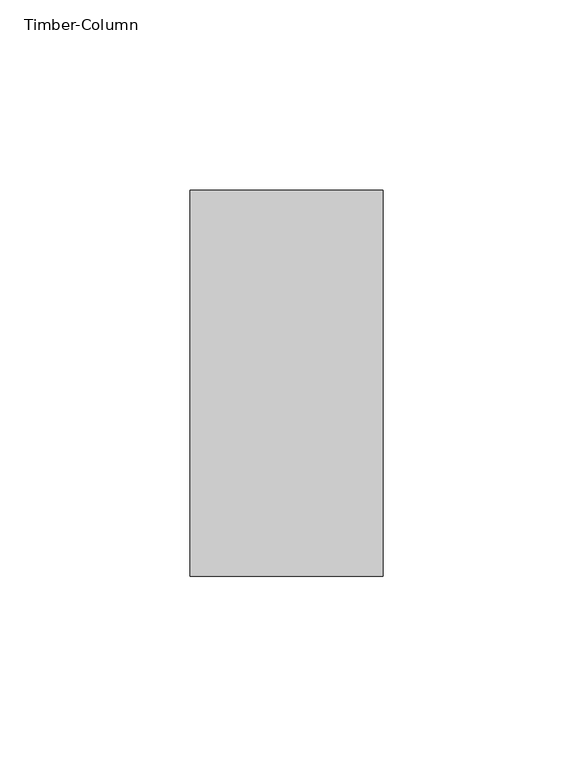
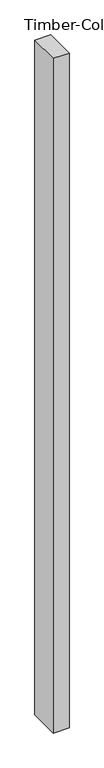
"""IFC4 building model written with IfcOpenShell, lengths in millimetres: column geometry, Timber-Column."""

from ifc_helpers import new_model, si_unit, frame, origin, place, context, project, spatial, polyline, outline, extrude, source, transform, mapped, element, save


def timber_column_b6a9144e(model_context):
    return source(origin(), model_context, "Body", "SweptSolid", [
        extrude(outline(polyline([(25.4, 50.8), (25.4, -50.8), (-25.4, -50.8), (-25.4, 50.8), (25.4, 50.8)])), frame((0.0, 0.0, 50.8), z_axis=(0.0, 0.0, 1.0), x_axis=(1.0, 0.0, 0.0)), (0.0, 0.0, 1.0), 2290.1727203),
    ])


if __name__ == "__main__":
    model = new_model("IFC4")
    model_context = context("Model", 3, world=origin())
    ifc_project = project(units=[si_unit("LENGTHUNIT", "METRE", prefix="MILLI")], contexts=[model_context])
    site = spatial("IfcSite", under=ifc_project)
    building = spatial("IfcBuilding", under=site)
    placement = place(None, origin())
    timber_column_shape = timber_column_b6a9144e(model_context)
    element("IfcColumn", 1, ObjectType="Timber-Column : BLDG 6241 Wall Struds 2\"x4\"", at=placement, inside=building, context=model_context, shape_type="MappedRepresentation", body=[
        mapped(timber_column_shape, transform((0.0, 0.0, 0.0), x_axis=(1.0, 0.0, 0.0), y_axis=(0.0, 1.0, 0.0), z_axis=(0.0, 0.0, 1.0))),
    ])
    save(model, "model.ifc")

# Revit data of these elements
# Type "Timber-Column : BLDG 6241 Wall Struds 2\"x4\""
#   Assembly Code = "B10"
#   A = 0.140625 SF
#   b = 0' - 2"
#   d = 0' - 4"
#   Structural Material [instance default] = Softwood, Lumber
# Element 1 (IfcColumn, "Timber-Column : BLDG 6241 Wall Struds 2\"x4\"")
#   Materials on its faces: "Softwood, Lumber"
# Materials
#   "Softwood, Lumber": class "Wood", colour RGB 223 192 134, transparency 0, Description = "Pinus Echinata", Cost = 0
